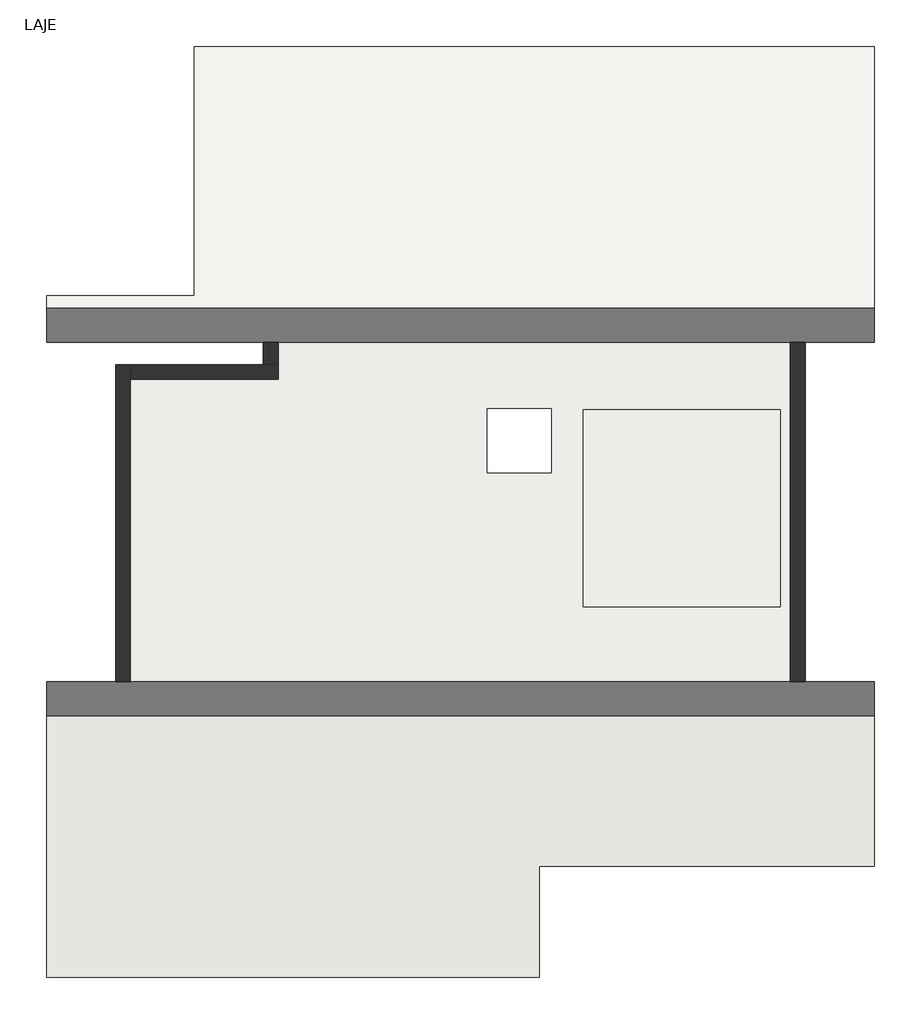
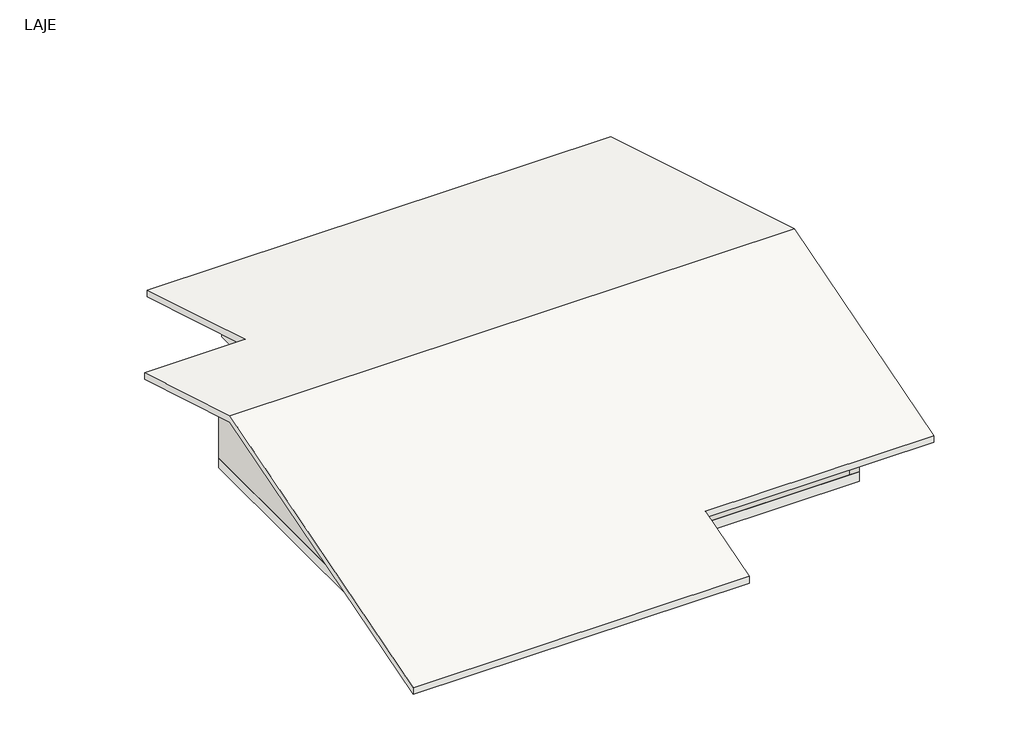
# One storey: 10 walls, 2 slabs, 1 roof.
"""IFC4 building model written with IfcOpenShell, lengths in millimetres."""

from ifc_helpers import new_model, si_unit, frame, origin, place, context, project, spatial, polyline, outline, extrude, faceted_brep, element, save

model = new_model("IFC4")

# Units and contexts
model_context = context("Model", 3, world=origin())
ifc_project = project(units=[si_unit("LENGTHUNIT", "METRE", prefix="MILLI")], contexts=[model_context])

# Site, building, storey
site = spatial("IfcSite", under=ifc_project)
building = spatial("IfcBuilding", under=site)
storey = spatial("IfcBuildingStorey", under=building, Name="LAJE", Elevation=3200.0)

# Roof
placement = place(None, origin())
element("IfcRoof", 1, ObjectType="Genérico - 400mm", at=placement, inside=storey, context=model_context, shape_type="Brep", body=[
    faceted_brep([(984.5823086, -5011.906943, 3500.0), (-4015.4176914, -5011.906943, 3500.0), (-4015.4176914, -286.906943, 4917.5), (4384.5823086, -286.906943, 4917.5), (4384.5823086, -3881.906943, 3839.0), (984.5823086, -3881.906943, 3839.0), (-4015.4176914, 1908.093057, 4259.0), (-2515.4176914, 1908.093057, 4259.0), (-2515.4176914, 4438.093057, 3500.0), (4384.5823086, 4438.093057, 3500.0), (-4015.4176914, -5011.906943, 3604.4030651), (984.5823086, -5011.906943, 3604.4030651), (984.5823086, -3881.906943, 3943.4030651), (4384.5823086, -3881.906943, 3943.4030651), (4384.5823086, -286.906943, 5021.9030651), (-4015.4176914, -286.906943, 5021.9030651), (-2515.4176914, 1908.093057, 4363.4030651), (-4015.4176914, 1908.093057, 4363.4030651), (4384.5823086, 4438.093057, 3604.4030651), (-2515.4176914, 4438.093057, 3604.4030651)], [[[0, 1, 2, 3, 4, 5]], [[6, 7, 8, 9, 3, 2]], [[10, 11, 12, 13, 14, 15]], [[16, 17, 15, 14, 18, 19]], [[0, 11, 10, 1]], [[8, 19, 18, 9]], [[17, 16, 7, 6]], [[16, 19, 8, 7]], [[10, 15, 17, 6, 2, 1]], [[12, 11, 0, 5]], [[13, 12, 5, 4]], [[18, 14, 13, 4, 3, 9]]]),
])

# Slabs
element("IfcSlab", 2, ObjectType="Laje de concreto", at=placement, inside=storey, context=model_context, shape_type="SweptSolid", body=[
    extrude(outline(polyline([(-1815.4176914, 3738.093057), (3684.5823086, 3738.093057), (3684.5823086, -3181.906943), (284.5823086, -3181.906943), (284.5823086, -4311.906943), (-3315.4176914, -4311.906943), (-3315.4176914, 1208.093057), (-1815.4176914, 1208.093057), (-1815.4176914, 3738.093057)]), holes=[polyline([(459.1823086, 112.693057), (1109.9823086, 112.693057), (1109.9823086, 763.493057), (459.1823086, 763.493057), (459.1823086, 112.693057)])]), frame((0.0, 0.0, 3050.0), z_axis=(0.0, 0.0, 1.0), x_axis=(1.0, 0.0, 0.0)), (0.0, 0.0, 1.0), 150.0),
])
element("IfcSlab", 3, ObjectType="Laje de concreto 15 cm", at=placement, inside=storey, context=model_context, shape_type="SweptSolid", body=[
    extrude(outline(polyline([(3434.5823086, 753.093057), (3434.5823086, -1246.906943), (1434.5823086, -1246.906943), (1434.5823086, 753.093057), (3434.5823086, 753.093057)])), frame((0.0, 0.0, 3670.0), z_axis=(0.0, 0.0, 1.0), x_axis=(1.0, 0.0, 0.0)), (0.0, 0.0, 1.0), 150.0),
])

# Walls
element("IfcWall", 4, ObjectType="Parede 15 cm - Genérica", at=placement, inside=storey, context=model_context, shape_type="SweptSolid", body=[
    extrude(outline(polyline([(1434.5823086, 753.093057), (3434.5823086, 753.093057), (3434.5823086, 603.093057), (1434.5823086, 603.093057), (1434.5823086, 753.093057)])), frame((0.0, 0.0, 3200.0), z_axis=(0.0, 0.0, 1.0), x_axis=(1.0, 0.0, 0.0)), (0.0, 0.0, 1.0), 470.0),
])
element("IfcWall", 5, ObjectType="Parede 15 cm - Genérica", at=placement, inside=storey, context=model_context, shape_type="SweptSolid", body=[
    extrude(outline(polyline([(1434.5823086, -1096.906943), (3434.5823086, -1096.906943), (3434.5823086, -1246.906943), (1434.5823086, -1246.906943), (1434.5823086, -1096.906943)])), frame((0.0, 0.0, 3200.0), z_axis=(0.0, 0.0, 1.0), x_axis=(1.0, 0.0, 0.0)), (0.0, 0.0, 1.0), 470.0),
])
element("IfcWall", 6, ObjectType="Parede 15 cm - Genérica", at=placement, inside=storey, context=model_context, shape_type="Brep", body=[
    faceted_brep([(284.5823086, -4161.906943, 3200.0), (134.5823086, -4161.906943, 3200.0), (-3165.4176914, -4161.906943, 3200.0), (-3315.4176914, -4161.906943, 3200.0), (-3315.4176914, -4161.906943, 3755.0), (-3165.4176914, -4161.906943, 3755.0), (134.5823086, -4161.906943, 3755.0), (284.5823086, -4161.906943, 3755.0), (284.5823086, -4311.906943, 3200.0), (284.5823086, -4311.906943, 3710.0), (-3315.4176914, -4311.906943, 3710.0), (-3315.4176914, -4311.906943, 3200.0)], [[[0, 1, 2, 3, 4, 5, 6, 7]], [[8, 9, 10, 11]], [[3, 2, 1, 0, 8, 11]], [[4, 3, 11, 10]], [[0, 7, 9, 8]], [[7, 6, 5, 4, 10, 9]]]),
])
element("IfcWall", 7, ObjectType="Parede 15 cm - Genérica", at=placement, inside=storey, context=model_context, shape_type="Brep", body=[
    faceted_brep([(-3165.4176914, -4161.906943, 3200.0), (-3165.4176914, 1058.093057, 3200.0), (-3165.4176914, 1208.093057, 3200.0), (-3165.4176914, 1208.093057, 4469.0), (-3165.4176914, 1058.093057, 4514.0), (-3165.4176914, -286.906943, 4917.5), (-3165.4176914, -4161.906943, 3755.0), (-3315.4176914, -4161.906943, 3200.0), (-3315.4176914, -4161.906943, 3755.0), (-3315.4176914, -286.906943, 4917.5), (-3315.4176914, 1208.093057, 4469.0), (-3315.4176914, 1208.093057, 3200.0)], [[[0, 1, 2, 3, 4, 5, 6]], [[7, 8, 9, 10, 11]], [[2, 1, 0, 7, 11]], [[0, 6, 8, 7]], [[3, 2, 11, 10]], [[6, 5, 9, 8]], [[5, 4, 3, 10, 9]]]),
])
element("IfcWall", 8, ObjectType="Parede 15 cm - Genérica", at=placement, inside=storey, context=model_context, shape_type="Brep", body=[
    faceted_brep([(-3165.4176914, 1058.093057, 3200.0), (-1665.4176914, 1058.093057, 3200.0), (-1665.4176914, 1058.093057, 4514.0), (-3165.4176914, 1058.093057, 4514.0), (-3165.4176914, 1208.093057, 3200.0), (-3165.4176914, 1208.093057, 4469.0), (-1815.4176914, 1208.093057, 4469.0), (-1665.4176914, 1208.093057, 4469.0), (-1665.4176914, 1208.093057, 3200.0), (-1815.4176914, 1208.093057, 3200.0)], [[[0, 1, 2, 3]], [[4, 5, 6, 7, 8, 9]], [[1, 0, 4, 9, 8]], [[0, 3, 5, 4]], [[2, 1, 8, 7]], [[3, 2, 7, 6, 5]]]),
])
element("IfcWall", 9, ObjectType="Parede 15 cm - Genérica", at=placement, inside=storey, context=model_context, shape_type="Brep", body=[
    faceted_brep([(-1665.4176914, 1208.093057, 3200.0), (-1665.4176914, 3588.093057, 3200.0), (-1665.4176914, 3738.093057, 3200.0), (-1665.4176914, 3738.093057, 3710.0), (-1665.4176914, 3588.093057, 3755.0), (-1665.4176914, 1208.093057, 4469.0), (-1815.4176914, 1208.093057, 3200.0), (-1815.4176914, 1208.093057, 4469.0), (-1815.4176914, 3738.093057, 3710.0), (-1815.4176914, 3738.093057, 3200.0)], [[[0, 1, 2, 3, 4, 5]], [[6, 7, 8, 9]], [[2, 1, 0, 6, 9]], [[0, 5, 7, 6]], [[3, 2, 9, 8]], [[5, 4, 3, 8, 7]]]),
])
element("IfcWall", 10, ObjectType="Parede 15 cm - Genérica", at=placement, inside=storey, context=model_context, shape_type="Brep", body=[
    faceted_brep([(-1665.4176914, 3588.093057, 3200.0), (3534.5823086, 3588.093057, 3200.0), (3684.5823086, 3588.093057, 3200.0), (3684.5823086, 3588.093057, 3755.0), (3534.5823086, 3588.093057, 3755.0), (-1665.4176914, 3588.093057, 3755.0), (-1665.4176914, 3738.093057, 3200.0), (-1665.4176914, 3738.093057, 3710.0), (3684.5823086, 3738.093057, 3710.0), (3684.5823086, 3738.093057, 3200.0)], [[[0, 1, 2, 3, 4, 5]], [[6, 7, 8, 9]], [[2, 1, 0, 6, 9]], [[0, 5, 7, 6]], [[3, 2, 9, 8]], [[5, 4, 3, 8, 7]]]),
])
element("IfcWall", 11, ObjectType="Parede 15 cm - Genérica", at=placement, inside=storey, context=model_context, shape_type="Brep", body=[
    faceted_brep([(3534.5823086, 3588.093057, 3200.0), (3534.5823086, -3031.906943, 3200.0), (3534.5823086, -3181.906943, 3200.0), (3534.5823086, -3181.906943, 4049.0), (3534.5823086, -3031.906943, 4094.0), (3534.5823086, -286.906943, 4917.5), (3534.5823086, 3588.093057, 3755.0), (3684.5823086, 3588.093057, 3200.0), (3684.5823086, 3588.093057, 3755.0), (3684.5823086, -286.906943, 4917.5), (3684.5823086, -3181.906943, 4049.0), (3684.5823086, -3181.906943, 3200.0)], [[[0, 1, 2, 3, 4, 5, 6]], [[7, 8, 9, 10, 11]], [[2, 1, 0, 7, 11]], [[0, 6, 8, 7]], [[3, 2, 11, 10]], [[6, 5, 9, 8]], [[5, 4, 3, 10, 9]]]),
])
element("IfcWall", 12, ObjectType="Parede 15 cm - Genérica", at=placement, inside=storey, context=model_context, shape_type="Brep", body=[
    faceted_brep([(3534.5823086, -3031.906943, 3200.0), (134.5823086, -3031.906943, 3200.0), (134.5823086, -3031.906943, 4094.0), (3534.5823086, -3031.906943, 4094.0), (3534.5823086, -3181.906943, 3200.0), (3534.5823086, -3181.906943, 4049.0), (284.5823086, -3181.906943, 4049.0), (134.5823086, -3181.906943, 4049.0), (134.5823086, -3181.906943, 3200.0), (284.5823086, -3181.906943, 3200.0)], [[[0, 1, 2, 3]], [[4, 5, 6, 7, 8, 9]], [[1, 0, 4, 9, 8]], [[0, 3, 5, 4]], [[2, 1, 8, 7]], [[3, 2, 7, 6, 5]]]),
])
element("IfcWall", 13, ObjectType="Parede 15 cm - Genérica", at=placement, inside=storey, context=model_context, shape_type="SweptSolid", body=[
    extrude(outline(polyline([(-3181.906943, 3200.0), (-4161.906943, 3200.0), (-4161.906943, 3755.0), (-3181.906943, 4049.0), (-3181.906943, 3200.0)])), frame((134.5823086, 0.0, 0.0), z_axis=(1.0, 0.0, 0.0), x_axis=(0.0, 1.0, 0.0)), (0.0, 0.0, 1.0), 150.0),
])

save(model, "model.ifc")

# Revit data of these elements
# Project information
#   Data de emissão do projeto = "Data de emissão"
#   Status do projeto = "Status do projeto"
#   Nome do cliente = "Proprietário"
#   Endereço do projeto = "RUA A - BLOCO A"
#   Nome do projeto = "CURSO REVIT PLANTA HUMANIZADA"
#   Número do projeto = "Número do projeto"
# Type "Genérico - 400mm"
#   Layers, outside or top first: 0.100 m "Telha - Cerâmica" (function 1)
# Type "Laje de concreto"
#   URL = "www.construir.arq.br"
#   Description = "Laje estrutural h = 15 cm em concreto moldado in loco"
#   Function = 0
#   Layers, outside or top first: 0.150 m "Concreto - Concreto concretado no local" (function 1)
# Type "Laje de concreto 15 cm"
#   URL = "www.construir.arq.br"
#   Description = "Laje estrutural h = 15 cm em concreto moldado in loco"
#   Type Mark = "10"
#   Function = 0
#   Layers, outside or top first: 0.010 m "Piso de massa pré-definida" (function 1); 0.140 m "Concreto - Concreto concretado no local" (function 1)
# Type "Parede 15 cm - Genérica"
#   Layers, outside or top first: 0.150 m "Genérico branco" (function 1)
# Element 1 (IfcRoof, "Genérico - 400mm")
#   built-in parameter 1001705 = 16.4761 (stored number, unit not read)
#   built-in parameter 1001701 = 0.984252 (stored number, unit not read)
#   built-in parameter 1001710 = 33615
#   Phase Created = Construção nova
#   Materials on its faces: "Telha - Cerâmica"
# Element 2 (IfcSlab, "Laje de concreto")
#   built-in parameter 1001955 = 3.14159 (stored number, unit not read)
#   Height Offset From Level = 0.000 m
#   Phase Created = Construção nova
#   Materials on its faces: "Concreto - Concreto concretado no local"
# Element 3 (IfcSlab, "Laje de concreto 15 cm")
#   Height Offset From Level = 0.620 m
#   Phase Created = Construção nova
#   Materials on its faces: "Concreto - Concreto concretado no local"
# Elements 4, 5 (IfcWall, "Parede 15 cm - Genérica")
#   Top Offset = 0.000 m
#   Base Offset = 0.000 m
#   Unconnected Height = 0.470 m
#   wall height = 0.470 m
#   Phase Created = Construção nova
#   Base Constraint = LAJE
#   Materials on its faces: "Genérico branco"
# Elements 6, 7, 8, 9, 10, 11, 12, 13 (IfcWall, "Parede 15 cm - Genérica")
#   Top Offset = 0.000 m
#   Base Offset = 0.000 m
#   Unconnected Height = 0.150 m
#   wall height = 0.150 m
#   Phase Created = Construção nova
#   Base Constraint = LAJE
#   Materials on its faces: "Genérico branco"
# Materials
#   "Telha - Cerâmica": class "Cerâmica", colour RGB 134 55 46, transparency 0, Description = "Interior finish", Cost = 0
#   "Concreto - Concreto concretado no local": class "Concreto", colour RGB 255 255 255, transparency 0, Description = "Rampa em Concreto armado e = 15cm i=29%", Cost = 0
#   "Piso de massa pré-definida": class "Diversos", colour RGB 122 75 31, transparency 0, Cost = 0
#   "Genérico branco": class "Parede drywall", colour RGB 244 244 244, transparency 0, Description = "Acabamento interno", Cost = 0
